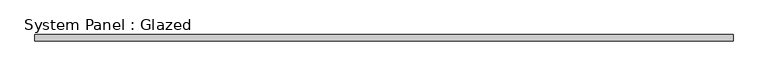
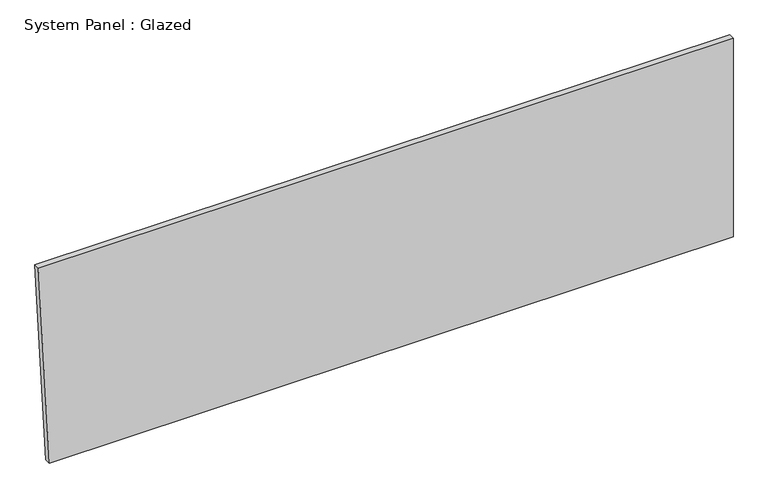
"""IFC4 building model written with IfcOpenShell, lengths in millimetres: plate geometry, System Panel : Glazed."""

from ifc_helpers import new_model, si_unit, frame, origin, place, context, project, spatial, polyline, outline, extrude, source, transform, mapped, element, save


def system_panel_glazed_b0ec51c6(model_context):
    return source(origin(), model_context, "Body", "SweptSolid", [
        extrude(outline(polyline([(0.0, -1389.0768125), (0.0, 1434.3998477), (866.0018549, 1434.3998477), (866.0018549, -1434.3998477), (0.0, -1389.0768125)])), frame((0.0, -44.45, 0.0), z_axis=(0.0, 1.0, 0.0), x_axis=(0.0, 0.0, 1.0)), (0.0, 0.0, 1.0), 25.4),
    ])


if __name__ == "__main__":
    model = new_model("IFC4")
    model_context = context("Model", 3, world=origin())
    ifc_project = project(units=[si_unit("LENGTHUNIT", "METRE", prefix="MILLI")], contexts=[model_context])
    site = spatial("IfcSite", under=ifc_project)
    building = spatial("IfcBuilding", under=site)
    placement = place(None, origin())
    system_panel_glazed_shape = system_panel_glazed_b0ec51c6(model_context)
    element("IfcPlate", 1, ObjectType="System Panel : Glazed", at=placement, inside=building, context=model_context, shape_type="MappedRepresentation", body=[
        mapped(system_panel_glazed_shape, transform((0.0, 0.0, 0.0), x_axis=(1.0, 0.0, 0.0), y_axis=(0.0, 1.0, 0.0), z_axis=(0.0, 0.0, 1.0))),
    ])
    save(model, "model.ifc")

# Revit data of these elements
# Type "System Panel : Glazed"
#   Construction Type Id = "GSP4R"
#   Analytic Construction = "1/8 in Pilkington single glazing"
#   Visual Light Transmittance = 0.9
#   Solar Heat Gain Coefficient = 0.86
#   Heat Transfer Coefficient (U) = 1.18115 BTU/(h·ft²·°F)
#   Define Thermal Properties by = 1
# Element 1 (IfcPlate, "System Panel : Glazed")
#   Materials on its faces: "Glass"
# Materials
#   "Glass": class "Glass", colour RGB 0 128 192, transparency 0.75, Description = "Soda Lime Glass", Cost = 0
